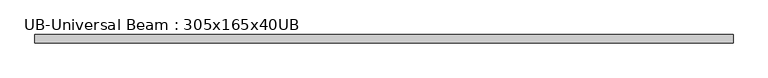
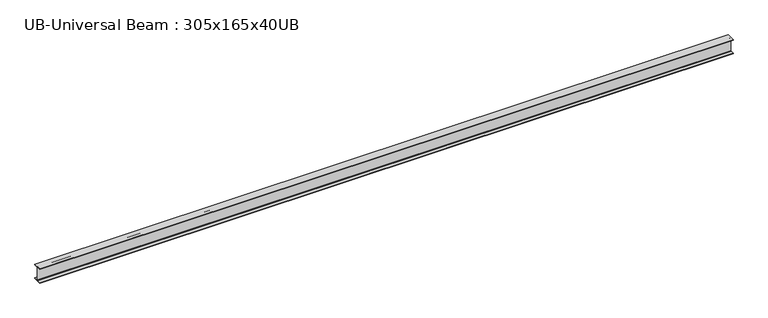
"""IFC4 building model written with IfcOpenShell, lengths in millimetres: beam geometry, UB-Universal Beam : 305x165x40UB."""

from ifc_helpers import new_model, si_unit, point, frame, frame_2d, origin, place, context, project, spatial, polyline, circle_curve, trimmed, segment, composite_curve, outline, extrude, source, transform, mapped, element, save


def ub_universal_beam_305x165x40ub_59300331(model_context):
    return source(origin(), model_context, "Body", "SweptSolid", [
        extrude(outline(composite_curve([segment(polyline([(82.5, -141.5), (82.5, -151.7), (-82.5, -151.7), (-82.5, -141.5), (-11.9, -141.5)]), True, "CONTINUOUS"), segment(trimmed(circle_curve(frame_2d((-11.9, -132.6)), 8.9), [point((-11.9, -141.5))], [point((-3.0, -132.6))], True, "CARTESIAN"), True, "CONTINUOUS"), segment(polyline([(-3.0, -132.6), (-3.0, 132.6)]), True, "CONTINUOUS"), segment(trimmed(circle_curve(frame_2d((-11.9, 132.6)), 8.9), [point((-3.0, 132.6))], [point((-11.9, 141.5))], True, "CARTESIAN"), True, "CONTINUOUS"), segment(polyline([(-11.9, 141.5), (-82.5, 141.5), (-82.5, 151.7), (82.5, 151.7), (82.5, 141.5), (11.9, 141.5)]), True, "CONTINUOUS"), segment(trimmed(circle_curve(frame_2d((11.9, 132.6)), 8.9), [point((11.9, 141.5))], [point((3.0, 132.6))], True, "CARTESIAN"), True, "CONTINUOUS"), segment(polyline([(3.0, 132.6), (3.0, -132.6)]), True, "CONTINUOUS"), segment(trimmed(circle_curve(frame_2d((11.9, -132.6)), 8.9), [point((3.0, -132.6))], [point((11.9, -141.5))], True, "CARTESIAN"), True, "CONTINUOUS"), segment(polyline([(11.9, -141.5), (82.5, -141.5)]), True, "CONTINUOUS")], self_intersect=False)), frame((-6958.35, 0.0, 0.0), z_axis=(1.0, 0.0, 0.0), x_axis=(0.0, 1.0, 0.0)), (0.0, 0.0, 1.0), 13916.7),
    ])


if __name__ == "__main__":
    model = new_model("IFC4")
    model_context = context("Model", 3, world=origin())
    ifc_project = project(units=[si_unit("LENGTHUNIT", "METRE", prefix="MILLI")], contexts=[model_context])
    site = spatial("IfcSite", under=ifc_project)
    building = spatial("IfcBuilding", under=site)
    placement = place(None, origin())
    ub_universal_beam_305x165x40ub_shape = ub_universal_beam_305x165x40ub_59300331(model_context)
    element("IfcBeam", 1, ObjectType="UB-Universal Beam : 305x165x40UB", at=placement, inside=building, context=model_context, shape_type="MappedRepresentation", body=[
        mapped(ub_universal_beam_305x165x40ub_shape, transform((0.0, 0.0, 0.0), x_axis=(1.0, 0.0, 0.0), y_axis=(0.0, 1.0, 0.0), z_axis=(0.0, 0.0, 1.0))),
    ])
    save(model, "model.ifc")

# Revit data of these elements
# Type "UB-Universal Beam : 305x165x40UB"
#   Nominal h = "305"
#   W = 0
#   Start Extension Calculation [instance default] = 3000 mm
#   Start Extension [instance default] = -12.7 mm
#   End Extension Calculation [instance default] = 3000 mm
#   End Extension [instance default] = -12.7 mm
#   Ix = 8503
#   Length [instance default] = 1524 mm
#   M = 40.3
#   Zx = 560
#   b = 165 mm
#   h = 303.4 mm
#   r = 8.9 mm
#   s = 6 mm
#   t = 10.2 mm
#   A = 0.005 m²
#   Structural Material [instance default] = Metal - Steel - 345 MPa
#   Assembly Code = ""
# Element 1 (IfcBeam, "UB-Universal Beam : 305x165x40UB")
#   Materials on its faces: "Metal - Steel - 345 MPa"
# Materials
#   "Metal - Steel - 345 MPa": class "Metal", colour RGB 241 46 46, transparency 0
